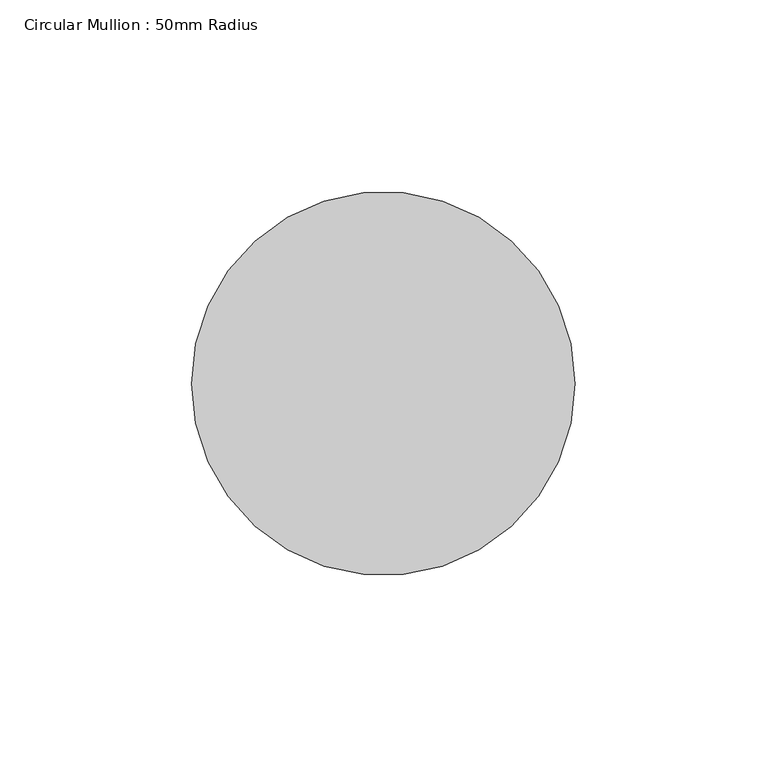
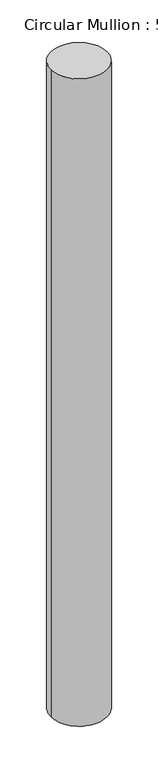
"""IFC4 building model written with IfcOpenShell, lengths in millimetres: member geometry, Circular Mullion : 50mm Radius."""

import ifcopenshell
import ifcopenshell.guid

model = None  # the IFC model being written
_history = None  # IfcOwnerHistory: only IFC2X3 demands one
_inside = {}  # id of a spatial element -> (the spatial element, [elements in it])
_under = {}  # id of a project, library or spatial element -> (it, [spatial elements below it])
_declared = {}  # id of a project -> (the project, [libraries it declares])
_typed = {}  # id of a type object -> (the type object, [elements of that type])
_made_of = {}  # id of a material, layer set ... -> (it, [elements and type objects made of it])


def new_model(schema):
    """Start an empty IFC model of exactly this schema.

    Asked for "IFC4X3", IfcOpenShell would pick the latest addendum, in which some entities
    have other attributes; the version numbers below select the first issue.
    IFC2X3 requires an IfcOwnerHistory on every rooted entity: one is made here for all.
    """
    global model, _history
    if schema == "IFC4X3":
        model = ifcopenshell.file(schema_version=(4, 3, 0, 0))
    else:
        model = ifcopenshell.file(schema=schema)
    _inside.clear()
    _under.clear()
    _declared.clear()
    _typed.clear()
    _made_of.clear()
    _history = None
    if model.schema == "IFC2X3":
        org = make("IfcOrganization", Name="unknown")
        user = make(
            "IfcPersonAndOrganization",
            ThePerson=make("IfcPerson", FamilyName="unknown"),
            TheOrganization=org,
        )
        app = make(
            "IfcApplication",
            ApplicationDeveloper=org,
            Version="unknown",
            ApplicationFullName="unknown",
            ApplicationIdentifier="unknown",
        )
        _history = make(
            "IfcOwnerHistory",
            OwningUser=user,
            OwningApplication=app,
            ChangeAction="ADDED",
            CreationDate=0,
        )
    return model


def make(cls, **values):
    """One entity of the class cls with the attributes given. An attribute that is None is left unset."""
    return model.create_entity(
        cls, **{name: value for name, value in values.items() if value is not None}
    )


def rooted(cls, **values):
    """An entity with a GlobalId (a new one), such as an element, a storey or a relation."""
    return make(cls, GlobalId=ifcopenshell.guid.new(), OwnerHistory=_history, **values)


def si_unit(unit_type, name, prefix=None):
    """IfcSIUnit, for example si_unit("LENGTHUNIT", "METRE", prefix="MILLI")."""
    return make("IfcSIUnit", UnitType=unit_type, Prefix=prefix, Name=name)


def assignment(units):
    """IfcUnitAssignment: the units of a project."""
    return None if units is None else make("IfcUnitAssignment", Units=units)


def point(xyz):
    """IfcCartesianPoint."""
    return None if xyz is None else make("IfcCartesianPoint", Coordinates=xyz)


def direction(xyz):
    """IfcDirection."""
    return None if xyz is None else make("IfcDirection", DirectionRatios=xyz)


def frame(location, z_axis=None, x_axis=None):
    """IfcAxis2Placement3D, a coordinate frame: its origin and axes. An axis left out is left unset."""
    return make(
        "IfcAxis2Placement3D",
        Location=point(location),
        Axis=direction(z_axis),
        RefDirection=direction(x_axis),
    )


def origin():
    """The frame at (0, 0, 0) with its axes left unset."""
    return frame((0.0, 0.0, 0.0))


def place(relative_to, where):
    """IfcLocalPlacement: puts the frame where relative to a parent placement (None: the world)."""
    return make(
        "IfcLocalPlacement", PlacementRelTo=relative_to, RelativePlacement=where
    )


def context(
    kind, dimensions, precision=None, world=None, true_north=None, identifier=None
):
    """IfcGeometricRepresentationContext, for example the 3D "Model" context."""
    return make(
        "IfcGeometricRepresentationContext",
        ContextIdentifier=identifier,
        ContextType=kind,
        CoordinateSpaceDimension=dimensions,
        Precision=precision,
        WorldCoordinateSystem=world,
        TrueNorth=true_north,
    )


def project(units=None, contexts=None):
    """IfcProject with its units and contexts."""
    return rooted(
        "IfcProject",
        Name="project",
        RepresentationContexts=contexts,
        UnitsInContext=assignment(units),
    )


def spatial(cls, under=None, at=None, **own):
    """A site, building, storey or space (cls), placed at a placement, below another one or the project."""
    s = rooted(cls, ObjectPlacement=at, **own)
    if under is not None:
        _under.setdefault(under.id(), (under, []))[1].append(s)
    return s


def ellipse_curve(where, semi_axis1, semi_axis2):
    """IfcEllipse in the frame where."""
    return make(
        "IfcEllipse", Position=where, SemiAxis1=semi_axis1, SemiAxis2=semi_axis2
    )


def shape(context_of_items, identifier, shape_type, items):
    """IfcShapeRepresentation: the items that make up one representation, for example the "Body"."""
    return make(
        "IfcShapeRepresentation",
        ContextOfItems=context_of_items,
        RepresentationIdentifier=identifier,
        RepresentationType=shape_type,
        Items=items,
    )


def source(mapping_origin, context_of_items, identifier, shape_type, items):
    """IfcRepresentationMap: a shape defined once, which mapped items show again and again."""
    return make(
        "IfcRepresentationMap",
        MappingOrigin=mapping_origin,
        MappedRepresentation=shape(context_of_items, identifier, shape_type, items),
    )


def transform(
    local_origin,
    x_axis=None,
    y_axis=None,
    z_axis=None,
    scale=None,
    scale2=None,
    scale3=None,
    uniform=True,
):
    """IfcCartesianTransformationOperator3D, or its non-uniform kind. x_axis, y_axis, z_axis: its Axis1, 2, 3."""
    if uniform:
        return make(
            "IfcCartesianTransformationOperator3D",
            Axis1=direction(x_axis),
            Axis2=direction(y_axis),
            LocalOrigin=point(local_origin),
            Scale=scale,
            Axis3=direction(z_axis),
        )
    return make(
        "IfcCartesianTransformationOperator3DnonUniform",
        Axis1=direction(x_axis),
        Axis2=direction(y_axis),
        LocalOrigin=point(local_origin),
        Scale=scale,
        Axis3=direction(z_axis),
        Scale2=scale2,
        Scale3=scale3,
    )


def mapped(mapping_source, mapping_target):
    """IfcMappedItem: shows the shape of a source again, moved by a transform."""
    return make(
        "IfcMappedItem", MappingSource=mapping_source, MappingTarget=mapping_target
    )


def made_of(thing, what):
    """Note that an element or type object is made of a material, layer set ...; save() writes the relation."""
    if what is not None:
        _made_of.setdefault(what.id(), (what, []))[1].append(thing)
    return thing


def element(
    cls,
    number,
    at=None,
    inside=None,
    cuts=None,
    type_object=None,
    material=None,
    context=None,
    identifier="Body",
    shape_type=None,
    held_by="IfcProductDefinitionShape",
    body=None,
    shapes=None,
    **own,
):
    """One element of the class cls, such as IfcWall. Its Tag is "e" and its number.

    at: its placement. inside: the storey or other place that contains it. cuts: it is an
    opening in that element (IfcRelVoidsElement). A single representation is given by context,
    identifier, shape_type and body (its items); several are given by shapes. held_by: the class
    of the entity that holds the representations. save() writes the other relations.
    """
    e = rooted(cls, Tag="e%d" % number, ObjectPlacement=at, **own)
    if body is not None:
        shapes = [shape(context, identifier, shape_type, body)]
    if shapes is not None:
        e.Representation = make(held_by, Representations=shapes)
    if inside is not None:
        _inside.setdefault(inside.id(), (inside, []))[1].append(e)
    if cuts is not None:
        rooted(
            "IfcRelVoidsElement", RelatingBuildingElement=cuts, RelatedOpeningElement=e
        )
    if type_object is not None:
        _typed.setdefault(type_object.id(), (type_object, []))[1].append(e)
    return made_of(e, material)


def aggregate(whole, parts):
    """IfcRelAggregates: a whole, such as a stair, and the parts it consists of."""
    return rooted("IfcRelAggregates", RelatingObject=whole, RelatedObjects=parts)


def save(model, path):
    """Write the relations noted so far, then the file.

    IfcRelAggregates (storeys below a building ...), IfcRelContainedInSpatialStructure (elements
    in a storey), IfcRelDefinesByType, IfcRelAssociatesMaterial and IfcRelDeclares: one each for
    every whole, place, type object, material and project.
    """
    for whole, parts in _under.values():
        aggregate(whole, parts)
    for where, things in _inside.values():
        rooted(
            "IfcRelContainedInSpatialStructure",
            RelatedElements=things,
            RelatingStructure=where,
        )
    for kind, things in _typed.values():
        rooted("IfcRelDefinesByType", RelatedObjects=things, RelatingType=kind)
    for what, things in _made_of.values():
        rooted("IfcRelAssociatesMaterial", RelatedObjects=things, RelatingMaterial=what)
    for by, libraries in _declared.values():
        rooted("IfcRelDeclares", RelatingContext=by, RelatedDefinitions=libraries)
    model.write(path)


def plane_surface(at):
    """IfcPlane: the flat surface through the origin of the frame at, square to its z axis."""
    return make("IfcPlane", Position=at)


def cylinder_surface(at, radius):
    """IfcCylindricalSurface: all points at the distance radius from the z axis of the frame at."""
    return make("IfcCylindricalSurface", Position=at, Radius=radius)


def advanced_brep(points, edges, surfaces, faces):
    """IfcAdvancedBrep: a solid bounded by faces that lie on surfaces and meet in shared edges.

    An edge is (start, end): straight between two places in points (the first is 0);
    or (start, end, curve); or (start, end, curve, False) where it runs against its curve.
    A face is (place in surfaces, loops), or (place, loops, False) where it looks against
    its surface's normal. A loop lists edges by number (the first is 1), with a minus sign
    where the edge is run from its end to its start. The first loop is the outer one.
    """
    corners = [point(p) for p in points]
    vertices = [make("IfcVertexPoint", VertexGeometry=c) for c in corners]
    made = []
    for start, end, *more in edges:
        made.append(
            make(
                "IfcEdgeCurve",
                EdgeStart=vertices[start],
                EdgeEnd=vertices[end],
                EdgeGeometry=more[0] if more else make("IfcPolyline", Points=[corners[start], corners[end]]),
                SameSense=more[1] if len(more) > 1 else True,
            )
        )
    hull = []
    for where, loops, *sense in faces:
        bounds = []
        for j, loop in enumerate(loops):
            ring = [make("IfcOrientedEdge", EdgeElement=made[abs(k) - 1], Orientation=k > 0) for k in loop]
            bounds.append(
                make(
                    "IfcFaceOuterBound" if j == 0 else "IfcFaceBound",
                    Bound=make("IfcEdgeLoop", EdgeList=ring),
                    Orientation=True,
                )
            )
        hull.append(make("IfcAdvancedFace", Bounds=bounds, FaceSurface=surfaces[where], SameSense=sense[0] if sense else True))
    return make("IfcAdvancedBrep", Outer=make("IfcClosedShell", CfsFaces=hull))


def circular_mullion_50mm_radius_1aa9b160(model_context):
    return source(origin(), model_context, "Body", "AdvancedBrep", [
        advanced_brep(
        [(-100.0, 0.0, 0.7478994), (0.0, 0.0, 0.0), (0.0, 0.0, -1216.4399189), (-100.0, 0.0, -1217.2197311)],
        [
            (0, 1, ellipse_curve(frame((-50.0, 0.0, 0.3739497), z_axis=(-0.007478124705351686, -0.013281386138172651, -0.9998838344693548), x_axis=(-0.49057026976326984, -0.8712683242592565, 0.015241967289684875)), 50.005809, 50.0)),
            (1, 2),
            (2, 3, ellipse_curve(frame((-50.0, 0.0, -1216.829825), z_axis=(-0.0077971375881346955, -0.013847963113847152, 0.9998737113070978), x_axis=(0.4905653030639354, 0.8712595032439066, 0.0158921816302931)), 50.0063152, 50.0)),
            (3, 0),
            (1, 0, ellipse_curve(frame((-50.0, 0.0, 0.3739497), z_axis=(-0.007478124705351686, -0.013281386138172651, -0.9998838344693548), x_axis=(-0.49057026976326984, -0.8712683242592565, 0.015241967289684875)), 50.005809, 50.0)),
            (3, 2, ellipse_curve(frame((-50.0, 0.0, -1216.829825), z_axis=(-0.0077971375881346955, -0.013847963113847152, 0.9998737113070978), x_axis=(0.4905653030639354, 0.8712595032439066, 0.0158921816302931)), 50.0063152, 50.0)),
        ],
        [
            cylinder_surface(frame((-50.0, 0.0, 0.0), z_axis=(0.0, 0.0, 1.0), x_axis=(1.0, 0.0, 0.0)), 50.0),
            plane_surface(frame((-265.593438, 149.54319, 0.0), z_axis=(0.007478124705351686, 0.013281386138172651, 0.9998838344693548), x_axis=(0.4905702697632712, 0.8712683242592556, -0.015241967289691835))),
            plane_surface(frame((-265.593438, 149.54319, -1216.4399189), z_axis=(0.0077971375881346955, 0.013847963113847152, -0.9998737113070978), x_axis=(0.4905653030639353, 0.8712595032439064, 0.015892181630310365))),
        ],
        [
            (0, [[1, 2, 3, 4]]),
            (0, [[5, -4, 6, -2]]),
            (1, [[-1, -5]]),
            (2, [[-6, -3]]),
        ],
    ),
    ])


if __name__ == "__main__":
    model = new_model("IFC4")
    model_context = context("Model", 3, world=origin())
    ifc_project = project(units=[si_unit("LENGTHUNIT", "METRE", prefix="MILLI")], contexts=[model_context])
    site = spatial("IfcSite", under=ifc_project)
    building = spatial("IfcBuilding", under=site)
    placement = place(None, origin())
    circular_mullion_50mm_radius_shape = circular_mullion_50mm_radius_1aa9b160(model_context)
    element("IfcMember", 1, ObjectType="Circular Mullion : 50mm Radius", at=placement, inside=building, context=model_context, shape_type="MappedRepresentation", body=[
        mapped(circular_mullion_50mm_radius_shape, transform((0.0, 0.0, 0.0), x_axis=(1.0, 0.0, 0.0), y_axis=(0.0, 1.0, 0.0), z_axis=(0.0, 0.0, 1.0))),
    ])
    save(model, "model.ifc")

# Revit data of these elements
# Type "Circular Mullion : 50mm Radius"
#   built-in parameter 1007350 = 0.164042 (stored number, unit not read)
# Element 1 (IfcMember, "Circular Mullion : 50mm Radius")
#   Materials on its faces: "Aluminium"
# Materials
#   "Aluminium": class "Metal", colour RGB 247 247 247, transparency 0, Description = "Aluminium 6061", Cost = 0
